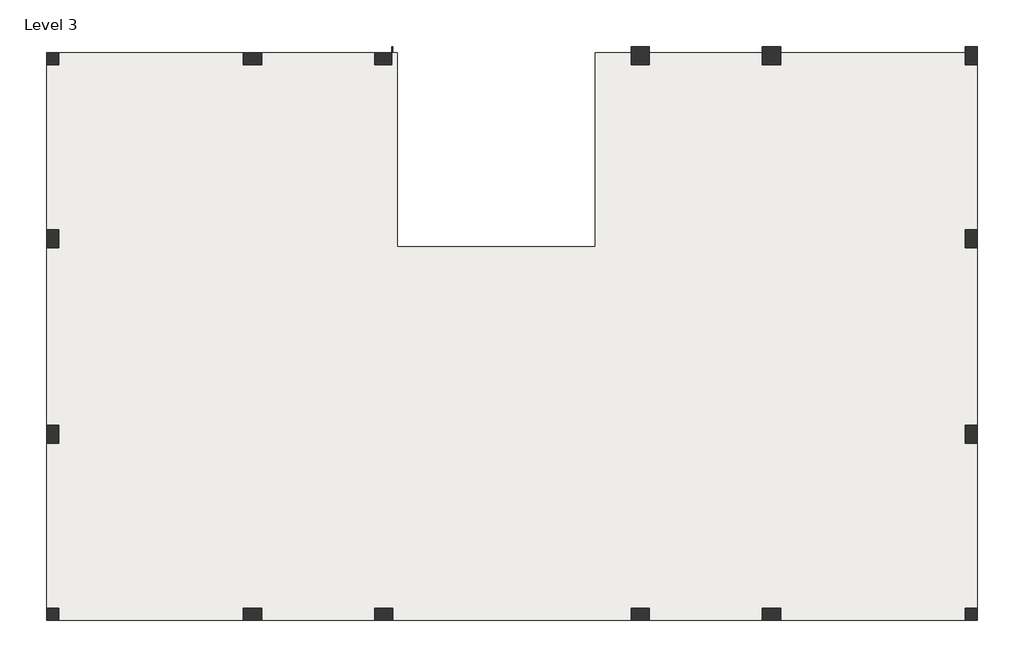
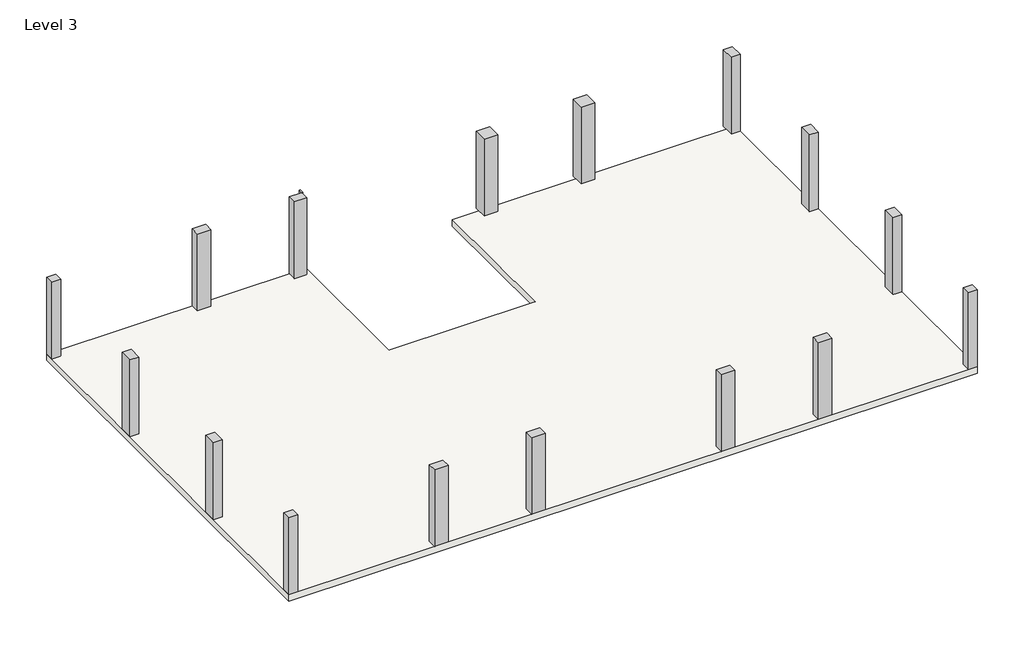
# One storey: 16 columns, 1 slab.
"""IFC4 building model written with IfcOpenShell, lengths in millimetres."""

import ifcopenshell
import ifcopenshell.guid

model = None  # the IFC model being written
_history = None  # IfcOwnerHistory: only IFC2X3 demands one
_inside = {}  # id of a spatial element -> (the spatial element, [elements in it])
_under = {}  # id of a project, library or spatial element -> (it, [spatial elements below it])
_declared = {}  # id of a project -> (the project, [libraries it declares])
_typed = {}  # id of a type object -> (the type object, [elements of that type])
_made_of = {}  # id of a material, layer set ... -> (it, [elements and type objects made of it])


def new_model(schema):
    """Start an empty IFC model of exactly this schema.

    Asked for "IFC4X3", IfcOpenShell would pick the latest addendum, in which some entities
    have other attributes; the version numbers below select the first issue.
    IFC2X3 requires an IfcOwnerHistory on every rooted entity: one is made here for all.
    """
    global model, _history
    if schema == "IFC4X3":
        model = ifcopenshell.file(schema_version=(4, 3, 0, 0))
    else:
        model = ifcopenshell.file(schema=schema)
    _inside.clear()
    _under.clear()
    _declared.clear()
    _typed.clear()
    _made_of.clear()
    _history = None
    if model.schema == "IFC2X3":
        org = make("IfcOrganization", Name="unknown")
        user = make(
            "IfcPersonAndOrganization",
            ThePerson=make("IfcPerson", FamilyName="unknown"),
            TheOrganization=org,
        )
        app = make(
            "IfcApplication",
            ApplicationDeveloper=org,
            Version="unknown",
            ApplicationFullName="unknown",
            ApplicationIdentifier="unknown",
        )
        _history = make(
            "IfcOwnerHistory",
            OwningUser=user,
            OwningApplication=app,
            ChangeAction="ADDED",
            CreationDate=0,
        )
    return model


def make(cls, **values):
    """One entity of the class cls with the attributes given. An attribute that is None is left unset."""
    return model.create_entity(
        cls, **{name: value for name, value in values.items() if value is not None}
    )


def rooted(cls, **values):
    """An entity with a GlobalId (a new one), such as an element, a storey or a relation."""
    return make(cls, GlobalId=ifcopenshell.guid.new(), OwnerHistory=_history, **values)


def si_unit(unit_type, name, prefix=None):
    """IfcSIUnit, for example si_unit("LENGTHUNIT", "METRE", prefix="MILLI")."""
    return make("IfcSIUnit", UnitType=unit_type, Prefix=prefix, Name=name)


def assignment(units):
    """IfcUnitAssignment: the units of a project."""
    return None if units is None else make("IfcUnitAssignment", Units=units)


def point(xyz):
    """IfcCartesianPoint."""
    return None if xyz is None else make("IfcCartesianPoint", Coordinates=xyz)


def direction(xyz):
    """IfcDirection."""
    return None if xyz is None else make("IfcDirection", DirectionRatios=xyz)


def frame(location, z_axis=None, x_axis=None):
    """IfcAxis2Placement3D, a coordinate frame: its origin and axes. An axis left out is left unset."""
    return make(
        "IfcAxis2Placement3D",
        Location=point(location),
        Axis=direction(z_axis),
        RefDirection=direction(x_axis),
    )


def origin():
    """The frame at (0, 0, 0) with its axes left unset."""
    return frame((0.0, 0.0, 0.0))


def place(relative_to, where):
    """IfcLocalPlacement: puts the frame where relative to a parent placement (None: the world)."""
    return make(
        "IfcLocalPlacement", PlacementRelTo=relative_to, RelativePlacement=where
    )


def context(
    kind, dimensions, precision=None, world=None, true_north=None, identifier=None
):
    """IfcGeometricRepresentationContext, for example the 3D "Model" context."""
    return make(
        "IfcGeometricRepresentationContext",
        ContextIdentifier=identifier,
        ContextType=kind,
        CoordinateSpaceDimension=dimensions,
        Precision=precision,
        WorldCoordinateSystem=world,
        TrueNorth=true_north,
    )


def project(units=None, contexts=None):
    """IfcProject with its units and contexts."""
    return rooted(
        "IfcProject",
        Name="project",
        RepresentationContexts=contexts,
        UnitsInContext=assignment(units),
    )


def spatial(cls, under=None, at=None, **own):
    """A site, building, storey or space (cls), placed at a placement, below another one or the project."""
    s = rooted(cls, ObjectPlacement=at, **own)
    if under is not None:
        _under.setdefault(under.id(), (under, []))[1].append(s)
    return s


def polyline(points):
    """IfcPolyline through the points."""
    return make("IfcPolyline", Points=[point(p) for p in points])


def outline(outer, holes=None, kind="AREA"):
    """IfcArbitraryClosedProfileDef: a profile drawn as a closed curve; with holes, ...WithVoids."""
    if holes is None:
        return make("IfcArbitraryClosedProfileDef", ProfileType=kind, OuterCurve=outer)
    return make(
        "IfcArbitraryProfileDefWithVoids",
        ProfileType=kind,
        OuterCurve=outer,
        InnerCurves=holes,
    )


def extrude(swept, where, along, depth):
    """IfcExtrudedAreaSolid: the profile swept, set in the frame where, extruded along a direction by depth."""
    return make(
        "IfcExtrudedAreaSolid",
        SweptArea=swept,
        Position=where,
        ExtrudedDirection=direction(along),
        Depth=depth,
    )


def shape(context_of_items, identifier, shape_type, items):
    """IfcShapeRepresentation: the items that make up one representation, for example the "Body"."""
    return make(
        "IfcShapeRepresentation",
        ContextOfItems=context_of_items,
        RepresentationIdentifier=identifier,
        RepresentationType=shape_type,
        Items=items,
    )


def made_of(thing, what):
    """Note that an element or type object is made of a material, layer set ...; save() writes the relation."""
    if what is not None:
        _made_of.setdefault(what.id(), (what, []))[1].append(thing)
    return thing


def element(
    cls,
    number,
    at=None,
    inside=None,
    cuts=None,
    type_object=None,
    material=None,
    context=None,
    identifier="Body",
    shape_type=None,
    held_by="IfcProductDefinitionShape",
    body=None,
    shapes=None,
    **own,
):
    """One element of the class cls, such as IfcWall. Its Tag is "e" and its number.

    at: its placement. inside: the storey or other place that contains it. cuts: it is an
    opening in that element (IfcRelVoidsElement). A single representation is given by context,
    identifier, shape_type and body (its items); several are given by shapes. held_by: the class
    of the entity that holds the representations. save() writes the other relations.
    """
    e = rooted(cls, Tag="e%d" % number, ObjectPlacement=at, **own)
    if body is not None:
        shapes = [shape(context, identifier, shape_type, body)]
    if shapes is not None:
        e.Representation = make(held_by, Representations=shapes)
    if inside is not None:
        _inside.setdefault(inside.id(), (inside, []))[1].append(e)
    if cuts is not None:
        rooted(
            "IfcRelVoidsElement", RelatingBuildingElement=cuts, RelatedOpeningElement=e
        )
    if type_object is not None:
        _typed.setdefault(type_object.id(), (type_object, []))[1].append(e)
    return made_of(e, material)


def aggregate(whole, parts):
    """IfcRelAggregates: a whole, such as a stair, and the parts it consists of."""
    return rooted("IfcRelAggregates", RelatingObject=whole, RelatedObjects=parts)


def save(model, path):
    """Write the relations noted so far, then the file.

    IfcRelAggregates (storeys below a building ...), IfcRelContainedInSpatialStructure (elements
    in a storey), IfcRelDefinesByType, IfcRelAssociatesMaterial and IfcRelDeclares: one each for
    every whole, place, type object, material and project.
    """
    for whole, parts in _under.values():
        aggregate(whole, parts)
    for where, things in _inside.values():
        rooted(
            "IfcRelContainedInSpatialStructure",
            RelatedElements=things,
            RelatingStructure=where,
        )
    for kind, things in _typed.values():
        rooted("IfcRelDefinesByType", RelatedObjects=things, RelatingType=kind)
    for what, things in _made_of.values():
        rooted("IfcRelAssociatesMaterial", RelatedObjects=things, RelatingMaterial=what)
    for by, libraries in _declared.values():
        rooted("IfcRelDeclares", RelatingContext=by, RelatedDefinitions=libraries)
    model.write(path)


model = new_model("IFC4")

# Units and contexts
model_context = context("Model", 3, world=origin())
ifc_project = project(units=[si_unit("LENGTHUNIT", "METRE", prefix="MILLI")], contexts=[model_context])

# Site, building, storey
site = spatial("IfcSite", under=ifc_project)
building = spatial("IfcBuilding", under=site)
storey = spatial("IfcBuildingStorey", under=building, Name="Level 3", Elevation=7315.2)

# Columns
placement = place(None, origin())
element("IfcColumn", 1, ObjectType="Rectangular Column : 24\" x 24\"", at=placement, inside=storey, context=model_context, shape_type="SweptSolid", body=[
    extrude(outline(polyline([(-16253.4122732, 9291.5015304), (-16253.4122732, 8885.1015304), (-16659.8122732, 8885.1015304), (-16659.8122732, 9291.5015304), (-16253.4122732, 9291.5015304)])), frame((0.0, 0.0, 7315.2), z_axis=(0.0, 0.0, 1.0), x_axis=(1.0, 0.0, 0.0)), (0.0, 0.0, 1.0), 3657.6),
])
element("IfcColumn", 2, ObjectType="Rectangular Column : 24\" x 24\"", at=placement, inside=storey, context=model_context, shape_type="SweptSolid", body=[
    extrude(outline(polyline([(-16253.4122732, 3398.7015304), (-16253.4122732, 2789.1015304), (-16659.8122732, 2789.1015304), (-16659.8122732, 3398.7015304), (-16253.4122732, 3398.7015304)])), frame((0.0, 0.0, 7315.2), z_axis=(0.0, 0.0, 1.0), x_axis=(1.0, 0.0, 0.0)), (0.0, 0.0, 1.0), 3657.6),
])
element("IfcColumn", 3, ObjectType="Rectangular Column : 24\" x 24\"", at=placement, inside=storey, context=model_context, shape_type="SweptSolid", body=[
    extrude(outline(polyline([(-9497.0122732, 8885.1015304), (-10106.6122732, 8885.1015304), (-10106.6122732, 9291.5015304), (-9497.0122732, 9291.5015304), (-9497.0122732, 8885.1015304)])), frame((0.0, 0.0, 7315.2), z_axis=(0.0, 0.0, 1.0), x_axis=(1.0, 0.0, 0.0)), (0.0, 0.0, 1.0), 3657.6),
])
element("IfcColumn", 4, ObjectType="Rectangular Column : 24\" x 24\"", at=placement, inside=storey, context=model_context, shape_type="SweptSolid", body=[
    extrude(outline(polyline([(-5174.2497732, 9494.7015304), (-5128.2122732, 9494.7015304), (-5128.2122732, 9301.0265304), (-5174.2497732, 9301.0265304), (-5174.2497732, 9494.7015304)])), frame((0.0, 0.0, 7315.2), z_axis=(0.0, 0.0, 1.0), x_axis=(1.0, 0.0, 0.0)), (0.0, 0.0, 1.0), 3657.6),
    extrude(outline(polyline([(-5737.8122732, 8885.1015304), (-5737.8122732, 9291.5015304), (-5174.2497732, 9291.5015304), (-5174.2497732, 8885.1015304), (-5737.8122732, 8885.1015304)])), frame((0.0, 0.0, 7315.2), z_axis=(0.0, 0.0, 1.0), x_axis=(1.0, 0.0, 0.0)), (0.0, 0.0, 1.0), 3657.6),
])
element("IfcColumn", 5, ObjectType="Rectangular Column : 24\" x 24\"", at=placement, inside=storey, context=model_context, shape_type="SweptSolid", body=[
    extrude(outline(polyline([(3406.1877268, 9494.7015304), (3406.1877268, 8885.1015304), (2796.5877268, 8885.1015304), (2796.5877268, 9494.7015304), (3406.1877268, 9494.7015304)])), frame((0.0, 0.0, 7315.2), z_axis=(0.0, 0.0, 1.0), x_axis=(1.0, 0.0, 0.0)), (0.0, 0.0, 1.0), 3657.6),
])
element("IfcColumn", 6, ObjectType="Rectangular Column : 24\" x 24\"", at=placement, inside=storey, context=model_context, shape_type="SweptSolid", body=[
    extrude(outline(polyline([(7774.9877268, 9494.7015304), (7774.9877268, 8885.1015304), (7165.3877268, 8885.1015304), (7165.3877268, 9494.7015304), (7774.9877268, 9494.7015304)])), frame((0.0, 0.0, 7315.2), z_axis=(0.0, 0.0, 1.0), x_axis=(1.0, 0.0, 0.0)), (0.0, 0.0, 1.0), 3657.6),
])
element("IfcColumn", 7, ObjectType="Rectangular Column : 24\" x 24\"", at=placement, inside=storey, context=model_context, shape_type="SweptSolid", body=[
    extrude(outline(polyline([(13921.7877268, 8885.1015304), (13921.7877268, 9494.7015304), (14328.1877268, 9494.7015304), (14328.1877268, 8885.1015304), (13921.7877268, 8885.1015304)])), frame((0.0, 0.0, 7315.2), z_axis=(0.0, 0.0, 1.0), x_axis=(1.0, 0.0, 0.0)), (0.0, 0.0, 1.0), 3657.6),
])
element("IfcColumn", 8, ObjectType="Rectangular Column : 24\" x 24\"", at=placement, inside=storey, context=model_context, shape_type="SweptSolid", body=[
    extrude(outline(polyline([(13921.7877268, 2789.1015304), (13921.7877268, 3398.7015304), (14328.1877268, 3398.7015304), (14328.1877268, 2789.1015304), (13921.7877268, 2789.1015304)])), frame((0.0, 0.0, 7315.2), z_axis=(0.0, 0.0, 1.0), x_axis=(1.0, 0.0, 0.0)), (0.0, 0.0, 1.0), 3657.6),
])
element("IfcColumn", 9, ObjectType="Rectangular Column : 24\" x 24\"", at=placement, inside=storey, context=model_context, shape_type="SweptSolid", body=[
    extrude(outline(polyline([(13921.7877268, -3713.2984696), (13921.7877268, -3103.6984696), (14328.1877268, -3103.6984696), (14328.1877268, -3713.2984696), (13921.7877268, -3713.2984696)])), frame((0.0, 0.0, 7315.2), z_axis=(0.0, 0.0, 1.0), x_axis=(1.0, 0.0, 0.0)), (0.0, 0.0, 1.0), 3657.6),
])
element("IfcColumn", 10, ObjectType="Rectangular Column : 24\" x 24\"", at=placement, inside=storey, context=model_context, shape_type="SweptSolid", body=[
    extrude(outline(polyline([(13921.7877268, -9606.0984696), (13921.7877268, -9199.6984696), (14328.1877268, -9199.6984696), (14328.1877268, -9606.0984696), (13921.7877268, -9606.0984696)])), frame((0.0, 0.0, 7315.2), z_axis=(0.0, 0.0, 1.0), x_axis=(1.0, 0.0, 0.0)), (0.0, 0.0, 1.0), 3657.6),
])
element("IfcColumn", 11, ObjectType="Rectangular Column : 24\" x 24\"", at=placement, inside=storey, context=model_context, shape_type="SweptSolid", body=[
    extrude(outline(polyline([(7165.3877268, -9199.6984696), (7774.9877268, -9199.6984696), (7774.9877268, -9606.0984696), (7165.3877268, -9606.0984696), (7165.3877268, -9199.6984696)])), frame((0.0, 0.0, 7315.2), z_axis=(0.0, 0.0, 1.0), x_axis=(1.0, 0.0, 0.0)), (0.0, 0.0, 1.0), 3657.6),
])
element("IfcColumn", 12, ObjectType="Rectangular Column : 24\" x 24\"", at=placement, inside=storey, context=model_context, shape_type="SweptSolid", body=[
    extrude(outline(polyline([(2796.5877268, -9199.6984696), (3406.1877268, -9199.6984696), (3406.1877268, -9606.0984696), (2796.5877268, -9606.0984696), (2796.5877268, -9199.6984696)])), frame((0.0, 0.0, 7315.2), z_axis=(0.0, 0.0, 1.0), x_axis=(1.0, 0.0, 0.0)), (0.0, 0.0, 1.0), 3657.6),
])
element("IfcColumn", 13, ObjectType="Rectangular Column : 24\" x 24\"", at=placement, inside=storey, context=model_context, shape_type="SweptSolid", body=[
    extrude(outline(polyline([(-5737.8122732, -9199.6984696), (-5128.2122732, -9199.6984696), (-5128.2122732, -9606.0984696), (-5737.8122732, -9606.0984696), (-5737.8122732, -9199.6984696)])), frame((0.0, 0.0, 7315.2), z_axis=(0.0, 0.0, 1.0), x_axis=(1.0, 0.0, 0.0)), (0.0, 0.0, 1.0), 3657.6),
])
element("IfcColumn", 14, ObjectType="Rectangular Column : 24\" x 24\"", at=placement, inside=storey, context=model_context, shape_type="SweptSolid", body=[
    extrude(outline(polyline([(-10106.6122732, -9199.6984696), (-9497.0122732, -9199.6984696), (-9497.0122732, -9606.0984696), (-10106.6122732, -9606.0984696), (-10106.6122732, -9199.6984696)])), frame((0.0, 0.0, 7315.2), z_axis=(0.0, 0.0, 1.0), x_axis=(1.0, 0.0, 0.0)), (0.0, 0.0, 1.0), 3657.6),
])
element("IfcColumn", 15, ObjectType="Rectangular Column : 24\" x 24\"", at=placement, inside=storey, context=model_context, shape_type="SweptSolid", body=[
    extrude(outline(polyline([(-16659.8122732, -9199.6984696), (-16253.4122732, -9199.6984696), (-16253.4122732, -9606.0984696), (-16659.8122732, -9606.0984696), (-16659.8122732, -9199.6984696)])), frame((0.0, 0.0, 7315.2), z_axis=(0.0, 0.0, 1.0), x_axis=(1.0, 0.0, 0.0)), (0.0, 0.0, 1.0), 3657.6),
])
element("IfcColumn", 16, ObjectType="Rectangular Column : 24\" x 24\"", at=placement, inside=storey, context=model_context, shape_type="SweptSolid", body=[
    extrude(outline(polyline([(-16253.4122732, -3103.6984696), (-16253.4122732, -3713.2984696), (-16659.8122732, -3713.2984696), (-16659.8122732, -3103.6984696), (-16253.4122732, -3103.6984696)])), frame((0.0, 0.0, 7315.2), z_axis=(0.0, 0.0, 1.0), x_axis=(1.0, 0.0, 0.0)), (0.0, 0.0, 1.0), 3657.6),
])

# Slab
element("IfcSlab", 17, ObjectType="Generic - 12\"", at=placement, inside=storey, context=model_context, shape_type="SweptSolid", body=[
    extrude(outline(polyline([(14328.1877268, 9291.5015304), (14328.1877268, -9606.0984696), (-16659.8122732, -9606.0984696), (-16659.8122732, 9291.5015304), (-4980.5747732, 9291.5015304), (-4980.5747732, 2835.1390304), (1602.7877268, 2835.1390304), (1602.7877268, 9291.5015304), (14328.1877268, 9291.5015304)])), frame((0.0, 0.0, 7010.4), z_axis=(0.0, 0.0, 1.0), x_axis=(1.0, 0.0, 0.0)), (0.0, 0.0, 1.0), 304.8),
])

save(model, "model.ifc")

# Revit data of these elements
# Type "Rectangular Column : 24\" x 24\""
#   Assembly Code = "B1010200"
#   Depth = 2' - 0"
#   Offset Base = 0' - 0"
#   Offset Top = 0' - 0"
#   Width = 2' - 0"
#   Material = none
# Type "Generic - 12\""
#   Assembly Code = "B1010"
#   Function = 0
#   Layers, outside or top first: 1' - 0" no material (function 1)
# Elements 1, 2, 3, 4, 7, 8, 9, 10, 11, 12, 13, 14, 15, 16 (IfcColumn, "Rectangular Column : 24\" x 24\"")
#   Phase Created = New Construction
#   Materials on its faces: "Default Wall"
# Elements 5, 6 (IfcColumn, "Rectangular Column : 24\" x 24\"")
#   Phase Created = New Construction
# Element 17 (IfcSlab, "Generic - 12\"")
#   built-in parameter 1001955 = 1.5708 (stored number, unit not read)
#   Height Offset From Level = 0' - 0"
#   Phase Created = New Construction
#   Materials on its faces: "Default Floor"
# Materials
#   "Default Wall": class "Miscellaneous", colour RGB 128 128 128, transparency 0, Cost = 0
#   "Default Floor": class "Miscellaneous", colour RGB 128 128 128, transparency 0, Cost = 0
